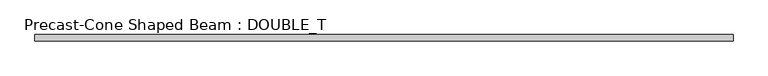
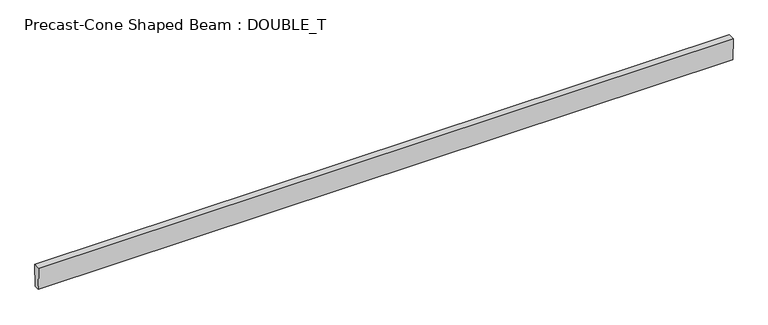
"""IFC4 building model written with IfcOpenShell, lengths in millimetres: beam geometry, Precast-Cone Shaped Beam : DOUBLE_T."""

from ifc_helpers import new_model, si_unit, frame, origin, place, context, project, spatial, polyline, outline, extrude, source, transform, mapped, element, save


def precast_cone_shaped_beam_double_t_383d5be5(model_context):
    return source(origin(), model_context, "Body", "SweptSolid", [
        extrude(outline(polyline([(50.8, -228.6), (-50.8, -228.6), (-63.5, 228.6), (63.5, 228.6), (50.8, -228.6)])), frame((-6930.23125, 0.0, 0.0), z_axis=(1.0, 0.0, 0.0), x_axis=(0.0, 1.0, 0.0)), (0.0, 0.0, 1.0), 13919.2),
    ])


if __name__ == "__main__":
    model = new_model("IFC4")
    model_context = context("Model", 3, world=origin())
    ifc_project = project(units=[si_unit("LENGTHUNIT", "METRE", prefix="MILLI")], contexts=[model_context])
    site = spatial("IfcSite", under=ifc_project)
    building = spatial("IfcBuilding", under=site)
    placement = place(None, origin())
    precast_cone_shaped_beam_double_t_shape = precast_cone_shaped_beam_double_t_383d5be5(model_context)
    element("IfcBeam", 1, ObjectType="Precast-Cone Shaped Beam : DOUBLE_T", at=placement, inside=building, context=model_context, shape_type="MappedRepresentation", body=[
        mapped(precast_cone_shaped_beam_double_t_shape, transform((0.0, 0.0, 0.0), x_axis=(1.0, 0.0, 0.0), y_axis=(0.0, 1.0, 0.0), z_axis=(0.0, 0.0, 1.0))),
    ])
    save(model, "model.ifc")

# Revit data of these elements
# Type "Precast-Cone Shaped Beam : DOUBLE_T"
#   Top Width = 0' - 5"
#   Tie Rod Weight [instance default] = 30
#   Tie Rod W [instance default] = 0.0660938 kip
#   Single Rebar Weight [instance default] = 50
#   Single Rebar W [instance default] = 0.110156 kip
#   Rebar Grids Weight [instance default] = 100
#   Rebar Grids W [instance default] = 0.220313 kip
#   Depth = 1' - 6"
#   Bottom Width = 0' - 4"
#   Length [instance default] = 5' - 0"
#   Structural Material [instance default] = Concrete, Precast
#   Assembly Code = ""
# Element 1 (IfcBeam, "Precast-Cone Shaped Beam : DOUBLE_T")
#   Length = 45' - 1 11/16"
#   Structural Material = Concrete - Precast Concrete - Normal Weight Concrete - 5 ksi
#   Materials on its faces: "Concrete - Precast Concrete - Normal Weight Concrete - 5 ksi"
# Materials
#   "Concrete, Precast": class "Concrete", colour RGB 198 187 187, transparency 0, Description = "Precast concrete", Cost = 0
#   "Concrete - Precast Concrete - Normal Weight Concrete - 5 ksi": class "Concrete", colour RGB 198 187 187, transparency 0, Cost = 0
